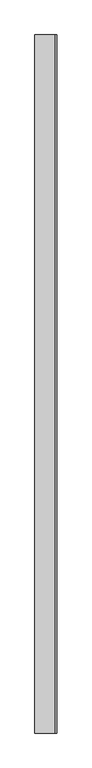
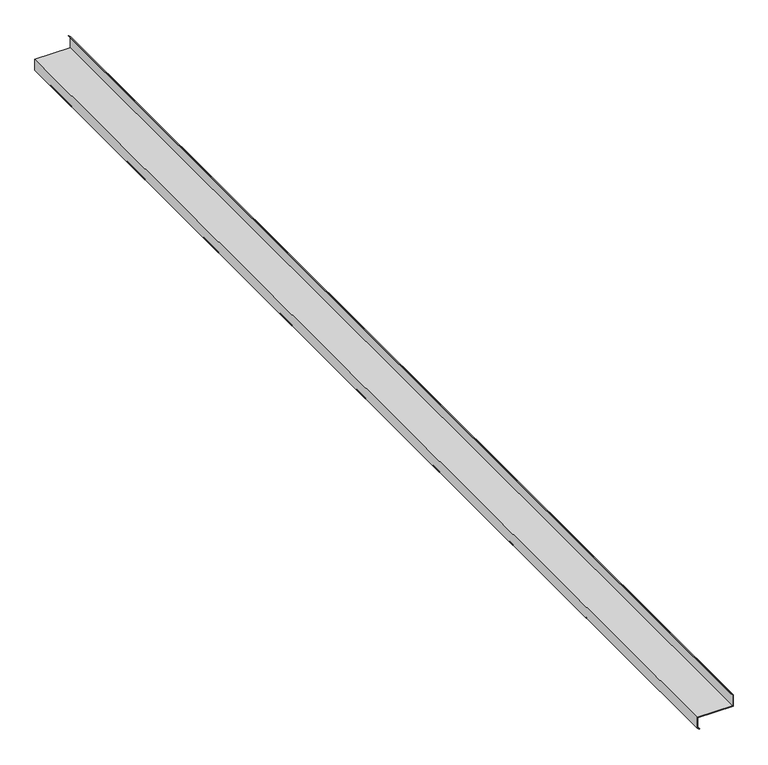
"""IFC4 building model written with IfcOpenShell, lengths in millimetres: proxy geometry, Generic Models 7:Generic Models 1:337419:Generic Models 1:337419 : Generic Models 7:Generic Models 1:337419:10 : Generic Models 7:Generic Models 1:337419:Generic Models 1:337419 : Generic Models 7:Generic Models 1:337419:301336."""

from ifc_helpers import new_model, si_unit, frame, origin, place, context, project, spatial, polyline, outline, extrude, source, transform, mapped, element, save


def generic_models_834b388e(model_context):
    return source(origin(), model_context, "Body", "SweptSolid", [
        extrude(outline(polyline([(208.5656924, 0.0), (208.5656924, -85.725), (194.1587363, -97.8138716), (192.1868015, -95.8419367), (205.7875674, -84.429539), (205.7875674, -2.778125), (-45.4343076, -2.778125), (-45.4343076, 76.596875), (-30.8411609, 88.841979), (-28.8692261, 86.8700441), (-42.6561826, 75.301414), (-42.6561826, 0.0), (208.5656924, 0.0)])), frame((578692.7460315, -568186.6413841, 6126.1625), z_axis=(1.98463467881993e-12, 1.0, 0.0), x_axis=(1.0, -1.98463467881993e-12, 0.0)), (0.0, 0.0, 1.0), 8141.4924408),
    ])


if __name__ == "__main__":
    model = new_model("IFC4")
    model_context = context("Model", 3, world=origin())
    ifc_project = project(units=[si_unit("LENGTHUNIT", "METRE", prefix="MILLI")], contexts=[model_context])
    site = spatial("IfcSite", under=ifc_project)
    building = spatial("IfcBuilding", under=site)
    placement = place(None, origin())
    generic_models_shape = generic_models_834b388e(model_context)
    element("IfcBuildingElementProxy", 1, Name="Generic Models 7:Generic Models 1:337419:Generic Models 1:337419 : Generic Models 7:Generic Models 1:337419:10 : Generic Models 7:Generic Models 1:337419:Generic Models 1:337419 : Generic Models 7:Generic Models 1:337419:301336", ObjectType="Generic Models 7:Generic Models 1:337419:Generic Models 1:337419 : Generic Models 7:Generic Models 1:337419:10 : Generic Models 7:Generic Models 1:337419:Generic Models 1:337419 : Generic Models 7:Generic Models 1:337419:301336", at=placement, inside=building, context=model_context, shape_type="MappedRepresentation", body=[
        mapped(generic_models_shape, transform((0.0, 0.0, 0.0), x_axis=(1.0, 0.0, 0.0), y_axis=(0.0, 1.0, 0.0), z_axis=(0.0, 0.0, 1.0))),
    ])
    save(model, "model.ifc")

# Revit data of these elements
# Type "Generic Models 7:Generic Models 1:337419:Generic Models 1:337419 : Generic Models 7:Generic Models 1:337419:10 : Generic Models 7:Generic Models 1:337419:Generic Models 1:337419 : Generic Models 7:Generic Models 1:337419:301336"
#   NameOverride = "Generic Models 7:Generic Models 1:337419:Generic Models 1:337419 : Generic Models 7:Generic Models 1:337419:301336"
#   ObjectTypeOverride = "Generic Models 1:337419 : Generic Models 7:Generic Models 1:337419"
#   Reference = "Generic Models 1"
#   Tag = "301336"
# Element 1 (IfcBuildingElementProxy, "Generic Models 7:Generic Models 1:337419:Generic Models 1:337419 : Generic Models 7:Generic Models 1:337419:10 : Generic Models 7:Generic Models 1:337419:Generic Models 1:337419 : Generic Models 7:Generic Models 1:337419:301336")
#   Materials on its faces: "'ZEE' SECTION (8.0x3.5Z - SEE STRUCT. DWGS)"
# Materials
#   "'ZEE' SECTION (8.0x3.5Z - SEE STRUCT. DWGS)": class "Unassigned", colour RGB 210 209 208, transparency 0, Keynote = "M05121300.02", Cost = 0
